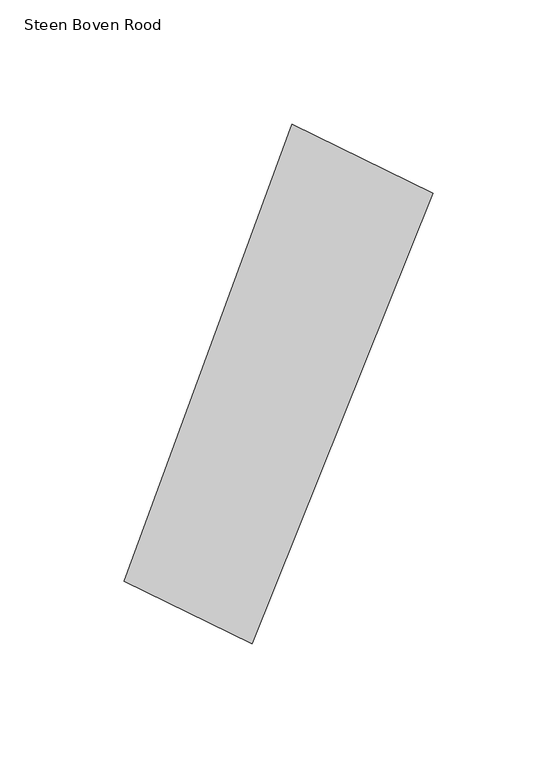
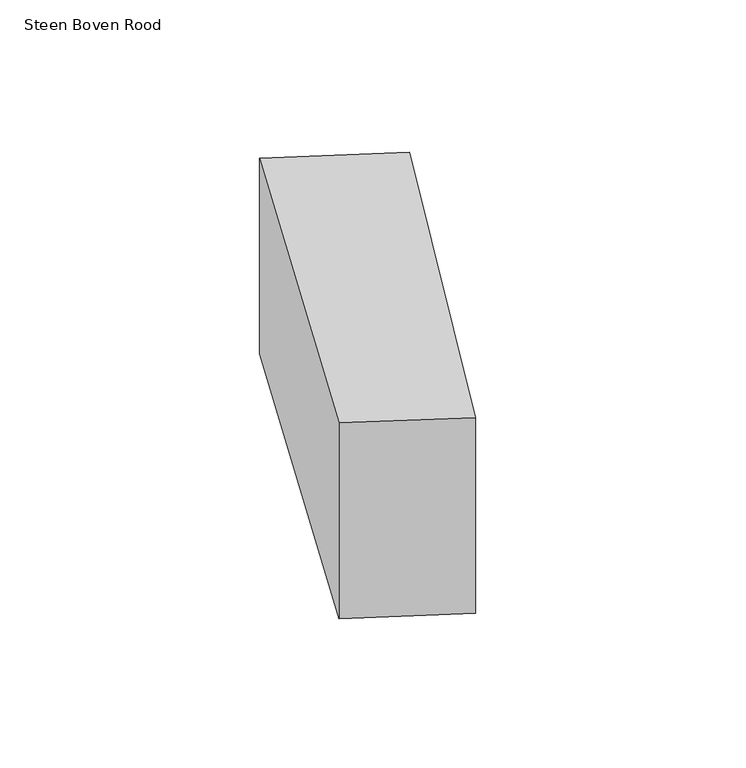
"""IFC4 building model written with IfcOpenShell, lengths in millimetres: proxy geometry, 00_GMA_steen_versie_4 : Steen Boven Rood."""

from ifc_helpers import new_model, si_unit, origin, origin_with_axes, place, context, project, spatial, polyline, outline, extrude, source, transform, mapped, element, save


def steen_boven_rood_74ba6ed9(model_context):
    return source(origin(), model_context, "Body", "SweptSolid", [
        extrude(outline(polyline([(138.4110375, 163.8424911), (65.573219, -17.6190617), (14.0218597, 7.5677502), (81.7419515, 191.5429047), (138.4110375, 163.8424911)])), origin_with_axes(), (0.0, 0.0, 1.0), 100.0),
    ])


if __name__ == "__main__":
    model = new_model("IFC4")
    model_context = context("Model", 3, world=origin())
    ifc_project = project(units=[si_unit("LENGTHUNIT", "METRE", prefix="MILLI")], contexts=[model_context])
    site = spatial("IfcSite", under=ifc_project)
    building = spatial("IfcBuilding", under=site)
    placement = place(None, origin())
    steen_boven_rood_shape = steen_boven_rood_74ba6ed9(model_context)
    element("IfcBuildingElementProxy", 1, Name="00_GMA_steen_versie_4 : Steen Boven Rood", ObjectType="00_GMA_steen_versie_4 : Steen Boven Rood", at=placement, inside=building, context=model_context, shape_type="MappedRepresentation", body=[
        mapped(steen_boven_rood_shape, transform((0.0, 0.0, 0.0), x_axis=(1.0, 0.0, 0.0), y_axis=(0.0, 1.0, 0.0), z_axis=(0.0, 0.0, 1.0))),
    ])
    save(model, "model.ifc")

# Revit data of these elements
# Type "00_GMA_steen_versie_4 : Steen Boven Rood"
#   StootVoegHalfBoven [instance default] = 5 mm
#   StootVoegHalf [instance default] = 5 mm
#   StootVoegBreedteOnder = 10 mm
#   StootVoegBreedteBoven = 10 mm
#   Steendikte = 100 mm
#   LintVoegOnderHalf = 5 mm
#   LintVoegOnder = 10 mm
#   LintVoegBovenHalf = 0 mm
#   LintVoegBoven = 0 mm
#   materiaal = 21_steen_rood
#   MateriaalVoeg = none
#   Default Elevation = 0
# Element 1 (IfcBuildingElementProxy, "00_GMA_steen_versie_4 : Steen Boven Rood")
#   Materials on its faces: "21_steen_rood"
# Materials
#   "21_steen_rood": class "Unassigned", colour RGB 213 111 43, transparency 0, Cost = 0
